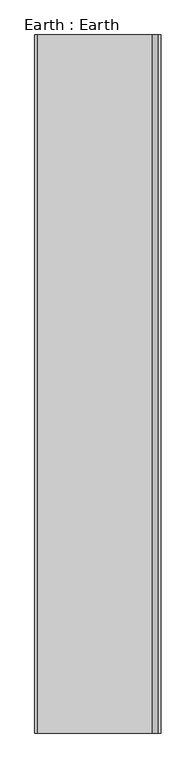
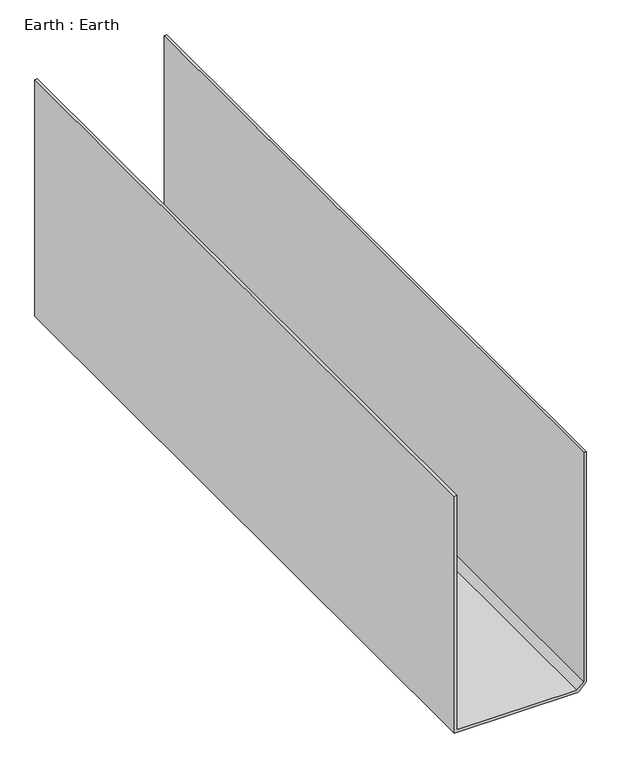
"""IFC4 building model written with IfcOpenShell, lengths in millimetres: proxy geometry, Earth : Earth."""

import ifcopenshell
import ifcopenshell.guid

model = None  # the IFC model being written
_history = None  # IfcOwnerHistory: only IFC2X3 demands one
_inside = {}  # id of a spatial element -> (the spatial element, [elements in it])
_under = {}  # id of a project, library or spatial element -> (it, [spatial elements below it])
_declared = {}  # id of a project -> (the project, [libraries it declares])
_typed = {}  # id of a type object -> (the type object, [elements of that type])
_made_of = {}  # id of a material, layer set ... -> (it, [elements and type objects made of it])


def new_model(schema):
    """Start an empty IFC model of exactly this schema.

    Asked for "IFC4X3", IfcOpenShell would pick the latest addendum, in which some entities
    have other attributes; the version numbers below select the first issue.
    IFC2X3 requires an IfcOwnerHistory on every rooted entity: one is made here for all.
    """
    global model, _history
    if schema == "IFC4X3":
        model = ifcopenshell.file(schema_version=(4, 3, 0, 0))
    else:
        model = ifcopenshell.file(schema=schema)
    _inside.clear()
    _under.clear()
    _declared.clear()
    _typed.clear()
    _made_of.clear()
    _history = None
    if model.schema == "IFC2X3":
        org = make("IfcOrganization", Name="unknown")
        user = make(
            "IfcPersonAndOrganization",
            ThePerson=make("IfcPerson", FamilyName="unknown"),
            TheOrganization=org,
        )
        app = make(
            "IfcApplication",
            ApplicationDeveloper=org,
            Version="unknown",
            ApplicationFullName="unknown",
            ApplicationIdentifier="unknown",
        )
        _history = make(
            "IfcOwnerHistory",
            OwningUser=user,
            OwningApplication=app,
            ChangeAction="ADDED",
            CreationDate=0,
        )
    return model


def make(cls, **values):
    """One entity of the class cls with the attributes given. An attribute that is None is left unset."""
    return model.create_entity(
        cls, **{name: value for name, value in values.items() if value is not None}
    )


def rooted(cls, **values):
    """An entity with a GlobalId (a new one), such as an element, a storey or a relation."""
    return make(cls, GlobalId=ifcopenshell.guid.new(), OwnerHistory=_history, **values)


def si_unit(unit_type, name, prefix=None):
    """IfcSIUnit, for example si_unit("LENGTHUNIT", "METRE", prefix="MILLI")."""
    return make("IfcSIUnit", UnitType=unit_type, Prefix=prefix, Name=name)


def assignment(units):
    """IfcUnitAssignment: the units of a project."""
    return None if units is None else make("IfcUnitAssignment", Units=units)


def point(xyz):
    """IfcCartesianPoint."""
    return None if xyz is None else make("IfcCartesianPoint", Coordinates=xyz)


def direction(xyz):
    """IfcDirection."""
    return None if xyz is None else make("IfcDirection", DirectionRatios=xyz)


def frame(location, z_axis=None, x_axis=None):
    """IfcAxis2Placement3D, a coordinate frame: its origin and axes. An axis left out is left unset."""
    return make(
        "IfcAxis2Placement3D",
        Location=point(location),
        Axis=direction(z_axis),
        RefDirection=direction(x_axis),
    )


def origin():
    """The frame at (0, 0, 0) with its axes left unset."""
    return frame((0.0, 0.0, 0.0))


def place(relative_to, where):
    """IfcLocalPlacement: puts the frame where relative to a parent placement (None: the world)."""
    return make(
        "IfcLocalPlacement", PlacementRelTo=relative_to, RelativePlacement=where
    )


def context(
    kind, dimensions, precision=None, world=None, true_north=None, identifier=None
):
    """IfcGeometricRepresentationContext, for example the 3D "Model" context."""
    return make(
        "IfcGeometricRepresentationContext",
        ContextIdentifier=identifier,
        ContextType=kind,
        CoordinateSpaceDimension=dimensions,
        Precision=precision,
        WorldCoordinateSystem=world,
        TrueNorth=true_north,
    )


def project(units=None, contexts=None):
    """IfcProject with its units and contexts."""
    return rooted(
        "IfcProject",
        Name="project",
        RepresentationContexts=contexts,
        UnitsInContext=assignment(units),
    )


def spatial(cls, under=None, at=None, **own):
    """A site, building, storey or space (cls), placed at a placement, below another one or the project."""
    s = rooted(cls, ObjectPlacement=at, **own)
    if under is not None:
        _under.setdefault(under.id(), (under, []))[1].append(s)
    return s


def polyline(points):
    """IfcPolyline through the points."""
    return make("IfcPolyline", Points=[point(p) for p in points])


def outline(outer, holes=None, kind="AREA"):
    """IfcArbitraryClosedProfileDef: a profile drawn as a closed curve; with holes, ...WithVoids."""
    if holes is None:
        return make("IfcArbitraryClosedProfileDef", ProfileType=kind, OuterCurve=outer)
    return make(
        "IfcArbitraryProfileDefWithVoids",
        ProfileType=kind,
        OuterCurve=outer,
        InnerCurves=holes,
    )


def extrude(swept, where, along, depth):
    """IfcExtrudedAreaSolid: the profile swept, set in the frame where, extruded along a direction by depth."""
    return make(
        "IfcExtrudedAreaSolid",
        SweptArea=swept,
        Position=where,
        ExtrudedDirection=direction(along),
        Depth=depth,
    )


def shape(context_of_items, identifier, shape_type, items):
    """IfcShapeRepresentation: the items that make up one representation, for example the "Body"."""
    return make(
        "IfcShapeRepresentation",
        ContextOfItems=context_of_items,
        RepresentationIdentifier=identifier,
        RepresentationType=shape_type,
        Items=items,
    )


def source(mapping_origin, context_of_items, identifier, shape_type, items):
    """IfcRepresentationMap: a shape defined once, which mapped items show again and again."""
    return make(
        "IfcRepresentationMap",
        MappingOrigin=mapping_origin,
        MappedRepresentation=shape(context_of_items, identifier, shape_type, items),
    )


def transform(
    local_origin,
    x_axis=None,
    y_axis=None,
    z_axis=None,
    scale=None,
    scale2=None,
    scale3=None,
    uniform=True,
):
    """IfcCartesianTransformationOperator3D, or its non-uniform kind. x_axis, y_axis, z_axis: its Axis1, 2, 3."""
    if uniform:
        return make(
            "IfcCartesianTransformationOperator3D",
            Axis1=direction(x_axis),
            Axis2=direction(y_axis),
            LocalOrigin=point(local_origin),
            Scale=scale,
            Axis3=direction(z_axis),
        )
    return make(
        "IfcCartesianTransformationOperator3DnonUniform",
        Axis1=direction(x_axis),
        Axis2=direction(y_axis),
        LocalOrigin=point(local_origin),
        Scale=scale,
        Axis3=direction(z_axis),
        Scale2=scale2,
        Scale3=scale3,
    )


def mapped(mapping_source, mapping_target):
    """IfcMappedItem: shows the shape of a source again, moved by a transform."""
    return make(
        "IfcMappedItem", MappingSource=mapping_source, MappingTarget=mapping_target
    )


def made_of(thing, what):
    """Note that an element or type object is made of a material, layer set ...; save() writes the relation."""
    if what is not None:
        _made_of.setdefault(what.id(), (what, []))[1].append(thing)
    return thing


def element(
    cls,
    number,
    at=None,
    inside=None,
    cuts=None,
    type_object=None,
    material=None,
    context=None,
    identifier="Body",
    shape_type=None,
    held_by="IfcProductDefinitionShape",
    body=None,
    shapes=None,
    **own,
):
    """One element of the class cls, such as IfcWall. Its Tag is "e" and its number.

    at: its placement. inside: the storey or other place that contains it. cuts: it is an
    opening in that element (IfcRelVoidsElement). A single representation is given by context,
    identifier, shape_type and body (its items); several are given by shapes. held_by: the class
    of the entity that holds the representations. save() writes the other relations.
    """
    e = rooted(cls, Tag="e%d" % number, ObjectPlacement=at, **own)
    if body is not None:
        shapes = [shape(context, identifier, shape_type, body)]
    if shapes is not None:
        e.Representation = make(held_by, Representations=shapes)
    if inside is not None:
        _inside.setdefault(inside.id(), (inside, []))[1].append(e)
    if cuts is not None:
        rooted(
            "IfcRelVoidsElement", RelatingBuildingElement=cuts, RelatedOpeningElement=e
        )
    if type_object is not None:
        _typed.setdefault(type_object.id(), (type_object, []))[1].append(e)
    return made_of(e, material)


def aggregate(whole, parts):
    """IfcRelAggregates: a whole, such as a stair, and the parts it consists of."""
    return rooted("IfcRelAggregates", RelatingObject=whole, RelatedObjects=parts)


def save(model, path):
    """Write the relations noted so far, then the file.

    IfcRelAggregates (storeys below a building ...), IfcRelContainedInSpatialStructure (elements
    in a storey), IfcRelDefinesByType, IfcRelAssociatesMaterial and IfcRelDeclares: one each for
    every whole, place, type object, material and project.
    """
    for whole, parts in _under.values():
        aggregate(whole, parts)
    for where, things in _inside.values():
        rooted(
            "IfcRelContainedInSpatialStructure",
            RelatedElements=things,
            RelatingStructure=where,
        )
    for kind, things in _typed.values():
        rooted("IfcRelDefinesByType", RelatedObjects=things, RelatingType=kind)
    for what, things in _made_of.values():
        rooted("IfcRelAssociatesMaterial", RelatedObjects=things, RelatingMaterial=what)
    for by, libraries in _declared.values():
        rooted("IfcRelDeclares", RelatingContext=by, RelatedDefinitions=libraries)
    model.write(path)


def earth_earth_d14d5190(model_context):
    return source(origin(), model_context, "Body", "SweptSolid", [
        extrude(outline(polyline([(32620.9902343, -10057.5706312), (32620.9902343, -9717.2148439), (32643.1028304, -9695.1022478), (33313.1445312, -9695.1022478), (33313.1445312, -9702.1022478), (32646.0023253, -9702.1022478), (32627.9902343, -9720.1143388), (32627.9902343, -10050.5706312), (33310.3609003, -10050.5706312), (33309.014262, -10057.5706312), (32620.9902343, -10057.5706312)])), frame((0.0, 7182.1531721, 0.0), z_axis=(0.0, 1.0, 0.0), x_axis=(0.0, 0.0, 1.0)), (0.0, 0.0, 1.0), 2000.0),
    ])


if __name__ == "__main__":
    model = new_model("IFC4")
    model_context = context("Model", 3, world=origin())
    ifc_project = project(units=[si_unit("LENGTHUNIT", "METRE", prefix="MILLI")], contexts=[model_context])
    site = spatial("IfcSite", under=ifc_project)
    building = spatial("IfcBuilding", under=site)
    placement = place(None, origin())
    earth_earth_shape = earth_earth_d14d5190(model_context)
    element("IfcBuildingElementProxy", 1, Name="Earth : Earth", ObjectType="Earth : Earth", at=placement, inside=building, context=model_context, shape_type="MappedRepresentation", body=[
        mapped(earth_earth_shape, transform((0.0, 0.0, 0.0), x_axis=(1.0, 0.0, 0.0), y_axis=(0.0, 1.0, 0.0), z_axis=(0.0, 0.0, 1.0))),
    ])
    save(model, "model.ifc")

# Revit data of these elements
# Type "Earth : Earth"
#   NameOverride = "Earth"
# Element 1 (IfcBuildingElementProxy, "Earth : Earth")
#   Materials on its faces: "WATERPROOF FIBER GLASS PLANTER LINER"
# Materials
#   "WATERPROOF FIBER GLASS PLANTER LINER": class "Unassigned", colour RGB 221 220 200, transparency 0, Cost = 0
